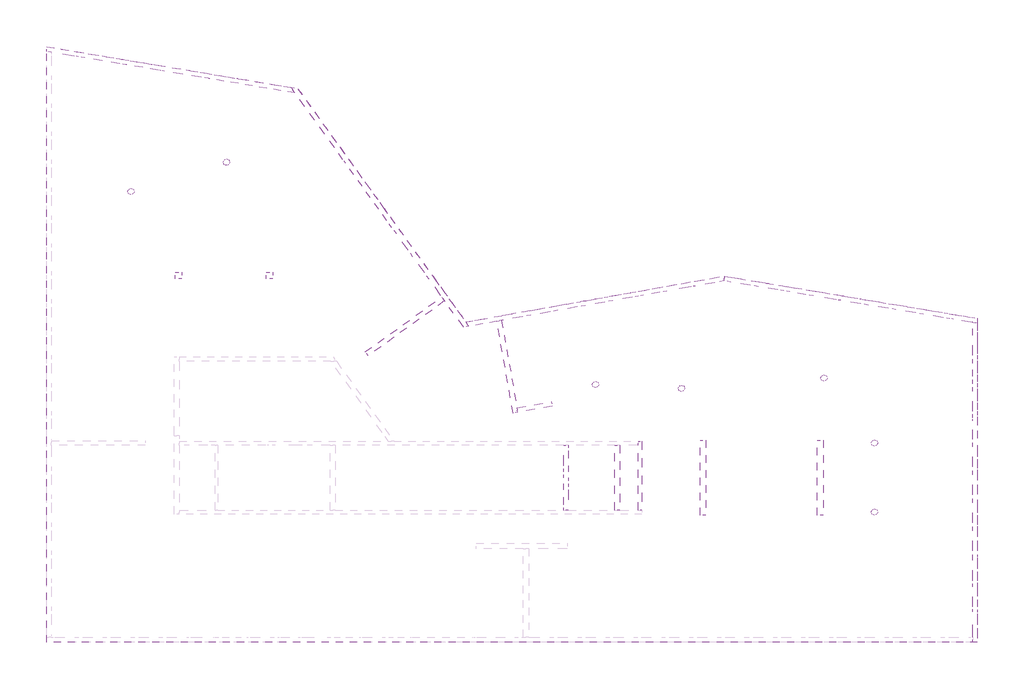
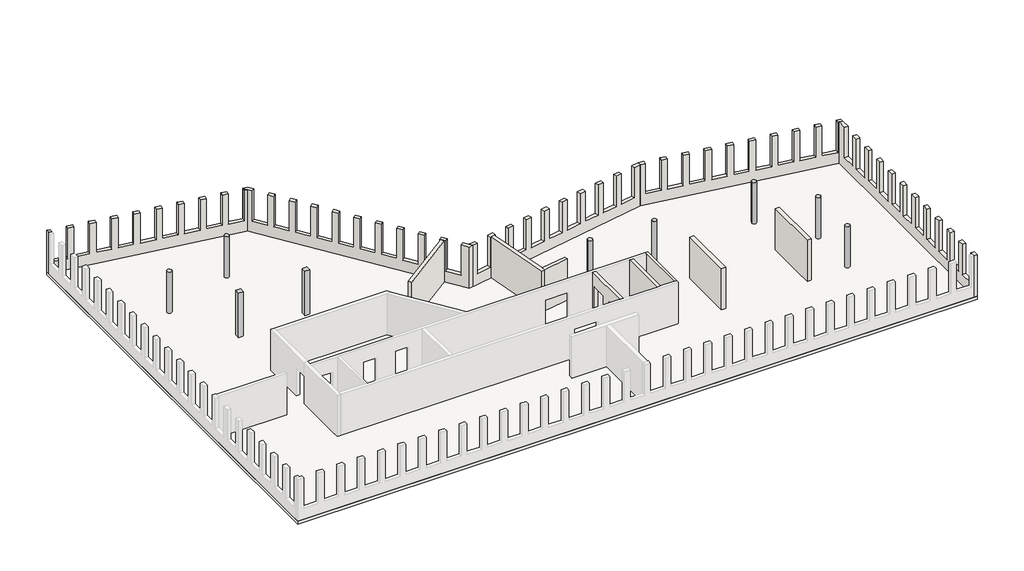
# One storey, part 2 of 2: 13 walls, 9 columns, 1 slab.
"""IFC4 building model written with IfcOpenShell, lengths in millimetres."""

from ifc_helpers import new_model, si_unit, point, frame, frame_2d, origin, place, context, project, spatial, polyline, circle_curve, trimmed, segment, composite_curve, outline, extrude, faceted_brep, element, save

model = new_model("IFC4")

# Units and contexts
model_context = context("Model", 3, world=origin())
ifc_project = project(units=[si_unit("LENGTHUNIT", "METRE", prefix="MILLI")], contexts=[model_context])

# Site, building, storey
site = spatial("IfcSite", under=ifc_project)
building = spatial("IfcBuilding", under=site)
storey = spatial("IfcBuildingStorey", under=building, Name="02_OG_OKFB_6,92", Elevation=6920.0)

# Columns
placement = place(None, origin())
element("IfcColumn", 1, ObjectType="5dki STB-Stützen rund : 5dki Stütze rund ø35cm C40/50", at=placement, inside=storey, context=model_context, shape_type="SweptSolid", body=[
    extrude(outline(composite_curve([segment(trimmed(circle_curve(frame_2d((33961.7583834, 13503.0230367)), 175.0), [point((34136.7583834, 13503.0230367))], [point((33786.7583834, 13503.0230367))], False, "CARTESIAN"), True, "CONTINUOUS"), segment(trimmed(circle_curve(frame_2d((33961.7583834, 13503.0230367)), 175.0), [point((33786.7583834, 13503.0230367))], [point((34136.7583834, 13503.0230367))], False, "CARTESIAN"), True, "CONTINUOUS")], self_intersect=False)), frame((0.0, 0.0, 10230.0), z_axis=(0.0, 0.0, 1.0), x_axis=(1.0, 0.0, 0.0)), (0.0, 0.0, 1.0), 3210.0),
])
element("IfcColumn", 2, ObjectType="5dki STB-Stützen rechteckig : 5dki Stütze recht. 35x35cm C35/45", at=placement, inside=storey, context=model_context, shape_type="SweptSolid", body=[
    extrude(outline(polyline([(7139.9999521, 19742.0124565), (7139.9999521, 19392.0124565), (6789.9999521, 19392.0124565), (6789.9999521, 19742.0124565), (7139.9999521, 19742.0124565)])), frame((0.0, 0.0, 10230.0), z_axis=(0.0, 0.0, 1.0), x_axis=(1.0, 0.0, 0.0)), (0.0, 0.0, 1.0), 3460.0),
])
element("IfcColumn", 3, ObjectType="5dki STB-Stützen rechteckig : 5dki Stütze recht. 35x35cm C35/45", at=placement, inside=storey, context=model_context, shape_type="SweptSolid", body=[
    extrude(outline(polyline([(12021.4450432, 19742.0124565), (12021.4450432, 19392.0124565), (11671.4450432, 19392.0124565), (11671.4450432, 19742.0124565), (12021.4450432, 19742.0124565)])), frame((0.0, 0.0, 10230.0), z_axis=(0.0, 0.0, 1.0), x_axis=(1.0, 0.0, 0.0)), (0.0, 0.0, 1.0), 3460.0),
])
element("IfcColumn", 4, ObjectType="5dki STB-Stützen rund : 5dki Stütze rund ø35cm C40/50", at=placement, inside=storey, context=model_context, shape_type="SweptSolid", body=[
    extrude(outline(composite_curve([segment(trimmed(circle_curve(frame_2d((41616.0718251, 14052.9332427)), 175.0), [point((41791.0718251, 14052.9332427))], [point((41441.0718251, 14052.9332427))], False, "CARTESIAN"), True, "CONTINUOUS"), segment(trimmed(circle_curve(frame_2d((41616.0718251, 14052.9332427)), 175.0), [point((41441.0718251, 14052.9332427))], [point((41791.0718251, 14052.9332427))], False, "CARTESIAN"), True, "CONTINUOUS")], self_intersect=False)), frame((0.0, 0.0, 10230.0), z_axis=(0.0, 0.0, 1.0), x_axis=(1.0, 0.0, 0.0)), (0.0, 0.0, 1.0), 3210.0),
])
element("IfcColumn", 5, ObjectType="5dki STB-Stützen rund : 5dki Stütze rund ø35cm C40/50", at=placement, inside=storey, context=model_context, shape_type="SweptSolid", body=[
    extrude(outline(composite_curve([segment(trimmed(circle_curve(frame_2d((44328.9990923, 10566.8309986)), 175.0), [point((44503.9990923, 10566.8309986))], [point((44153.9990923, 10566.8309986))], False, "CARTESIAN"), True, "CONTINUOUS"), segment(trimmed(circle_curve(frame_2d((44328.9990923, 10566.8309986)), 175.0), [point((44153.9990923, 10566.8309986))], [point((44503.9990923, 10566.8309986))], False, "CARTESIAN"), True, "CONTINUOUS")], self_intersect=False)), frame((0.0, 0.0, 10230.0), z_axis=(0.0, 0.0, 1.0), x_axis=(1.0, 0.0, 0.0)), (0.0, 0.0, 1.0), 3210.0),
])
element("IfcColumn", 6, ObjectType="5dki STB-Stützen rund : 5dki Stütze rund ø35cm C40/50", at=placement, inside=storey, context=model_context, shape_type="SweptSolid", body=[
    extrude(outline(composite_curve([segment(trimmed(circle_curve(frame_2d((44328.9990923, 6852.1619165)), 175.0), [point((44503.9990923, 6852.1619165))], [point((44153.9990923, 6852.1619165))], False, "CARTESIAN"), True, "CONTINUOUS"), segment(trimmed(circle_curve(frame_2d((44328.9990923, 6852.1619165)), 175.0), [point((44153.9990923, 6852.1619165))], [point((44503.9990923, 6852.1619165))], False, "CARTESIAN"), True, "CONTINUOUS")], self_intersect=False)), frame((0.0, 0.0, 10230.0), z_axis=(0.0, 0.0, 1.0), x_axis=(1.0, 0.0, 0.0)), (0.0, 0.0, 1.0), 3210.0),
])
element("IfcColumn", 7, ObjectType="5dki STB-Stützen rund : 5dki Stütze rund ø35cm C40/50", at=placement, inside=storey, context=model_context, shape_type="SweptSolid", body=[
    extrude(outline(composite_curve([segment(trimmed(circle_curve(frame_2d((9535.2710874, 25643.9282611)), 175.0), [point((9710.2710874, 25643.9282611))], [point((9360.2710874, 25643.9282611))], False, "CARTESIAN"), True, "CONTINUOUS"), segment(trimmed(circle_curve(frame_2d((9535.2710874, 25643.9282611)), 175.0), [point((9360.2710874, 25643.9282611))], [point((9710.2710874, 25643.9282611))], False, "CARTESIAN"), True, "CONTINUOUS")], self_intersect=False)), frame((0.0, 0.0, 10230.0), z_axis=(0.0, 0.0, 1.0), x_axis=(1.0, 0.0, 0.0)), (0.0, 0.0, 1.0), 3210.0),
])
element("IfcColumn", 8, ObjectType="5dki STB-Stützen rund : 5dki Stütze rund ø35cm C40/50", at=placement, inside=storey, context=model_context, shape_type="SweptSolid", body=[
    extrude(outline(composite_curve([segment(trimmed(circle_curve(frame_2d((4404.9034618, 24066.2757931)), 175.0), [point((4579.9034618, 24066.2757931))], [point((4229.9034618, 24066.2757931))], False, "CARTESIAN"), True, "CONTINUOUS"), segment(trimmed(circle_curve(frame_2d((4404.9034618, 24066.2757931)), 175.0), [point((4229.9034618, 24066.2757931))], [point((4579.9034618, 24066.2757931))], False, "CARTESIAN"), True, "CONTINUOUS")], self_intersect=False)), frame((0.0, 0.0, 10230.0), z_axis=(0.0, 0.0, 1.0), x_axis=(1.0, 0.0, 0.0)), (0.0, 0.0, 1.0), 3210.0),
])
element("IfcColumn", 9, ObjectType="5dki STB-Stützen rund : 5dki Stütze rund ø35cm C40/50", at=placement, inside=storey, context=model_context, shape_type="SweptSolid", body=[
    extrude(outline(composite_curve([segment(trimmed(circle_curve(frame_2d((29357.7423112, 13702.251654)), 175.0), [point((29532.7423112, 13702.251654))], [point((29182.7423112, 13702.251654))], False, "CARTESIAN"), True, "CONTINUOUS"), segment(trimmed(circle_curve(frame_2d((29357.7423112, 13702.251654)), 175.0), [point((29182.7423112, 13702.251654))], [point((29532.7423112, 13702.251654))], False, "CARTESIAN"), True, "CONTINUOUS")], self_intersect=False)), frame((0.0, 0.0, 10230.0), z_axis=(0.0, 0.0, 1.0), x_axis=(1.0, 0.0, 0.0)), (0.0, 0.0, 1.0), 3210.0),
])

# Slab
element("IfcSlab", 10, ObjectType="5dki Decke Ortbeton 25cm C30/37", at=placement, inside=storey, context=model_context, shape_type="SweptSolid", body=[
    extrude(outline(polyline([(-129.9989953, 31855.7150729), (13359.8955383, 29603.0549033), (22383.5041721, 17069.4128529), (36259.9888873, 19532.5499737), (49863.9990833, 17260.8337794), (49863.9991105, -129.9989509), (-129.9989953, -129.9990284), (-129.9989953, 31855.7150729)]), holes=[polyline([(30391.9999891, 10442.0127433), (27891.9999829, 10442.0127433), (27891.9999829, 6960.0000497), (30391.9999891, 6960.0000497), (30391.9999891, 10442.0127433)]), polyline([(31641.9999382, 10442.0127483), (30641.9999891, 10442.0127483), (30641.9999891, 6960.0000514), (31641.9999382, 6960.0000514), (31641.9999382, 10442.0127483)]), polyline([(8916.9999886, 10442.0127052), (6989.9995723, 10442.0127052), (6989.9995723, 6960.0000232), (8916.9999886, 6960.0000232), (8916.9999886, 10442.0127052)]), polyline([(24127.0004657, 8820.0328918), (16927.0004692, 8820.0328918), (16927.0004692, 7020.033352), (24127.0004657, 7020.033352), (24127.0004657, 8820.0328918)])]), frame((0.0, 0.0, 9980.0), z_axis=(0.0, 0.0, 1.0), x_axis=(1.0, 0.0, 0.0)), (0.0, 0.0, 1.0), 250.0),
])

# Walls
element("IfcWall", 11, ObjectType="5dki Lochfassade 26cm C30/37", at=placement, inside=storey, context=model_context, shape_type="Brep", body=[
    faceted_brep([(12995.7423601, 29663.864375, 10230.0), (13211.4553837, 29364.2425792, 10230.0), (22268.004401, 16784.8468851, 10230.0), (22268.004401, 16784.8468851, 13440.0), (21924.4906268, 17261.9817942, 13440.0), (21924.4906268, 17261.9817942, 11090.0), (21293.4697845, 18138.4592307, 11090.0), (21293.4697845, 18138.4592307, 13440.0), (21048.0727903, 18479.3115671, 13440.0), (21048.0727903, 18479.3115671, 11090.0), (20417.0519481, 19355.7890035, 11090.0), (20417.0519481, 19355.7890035, 13440.0), (20171.6549538, 19696.64134, 13440.0), (20171.6549538, 19696.64134, 11090.0), (19540.6341116, 20573.1187764, 11090.0), (19540.6341116, 20573.1187764, 13440.0), (19295.2371174, 20913.9711128, 13440.0), (19295.2371174, 20913.9711128, 11090.0), (18664.2162751, 21790.4485493, 11090.0), (18664.2162751, 21790.4485493, 13440.0), (18418.8192809, 22131.3008857, 13440.0), (18418.8192809, 22131.3008857, 11090.0), (17787.7984387, 23007.7783222, 11090.0), (17787.7984387, 23007.7783222, 13440.0), (17542.4014445, 23348.6306586, 13440.0), (17542.4014445, 23348.6306586, 11090.0), (16911.3806022, 24225.1080951, 11090.0), (16911.3806022, 24225.1080951, 13440.0), (16665.983608, 24565.9604315, 13440.0), (16665.983608, 24565.9604315, 11090.0), (16034.9627658, 25442.4378679, 11090.0), (16034.9627658, 25442.4378679, 13440.0), (15789.5657715, 25783.2902043, 13440.0), (15789.5657715, 25783.2902043, 11090.0), (15158.5449293, 26659.7676408, 11090.0), (15158.5449293, 26659.7676408, 13440.0), (14913.1479351, 27000.6199772, 13440.0), (14913.1479351, 27000.6199772, 11090.0), (14282.1270928, 27877.0974137, 11090.0), (14282.1270928, 27877.0974137, 13440.0), (14036.7300986, 28217.9497501, 13440.0), (14036.7300986, 28217.9497501, 11090.0), (13405.7092564, 29094.4271866, 11090.0), (13405.7092564, 29094.4271866, 13440.0), (13211.4553837, 29364.2425792, 13440.0), (13028.1664453, 29618.8278609, 13440.0), (13028.1664453, 29618.8278609, 11090.0), (12995.7423601, 29663.864375, 11090.0), (22552.0750732, 16835.2706799, 10230.0), (22383.5041721, 17069.4128529, 10230.0), (13359.8955383, 29603.0549033, 10230.0), (13359.8955383, 29603.0549033, 13440.0), (13616.7130837, 29246.3396115, 13440.0), (13616.7130837, 29246.3396115, 11090.0), (14247.7339259, 28369.8621751, 11090.0), (14247.7339259, 28369.8621751, 13440.0), (14493.1309201, 28029.0098387, 13440.0), (14493.1309201, 28029.0098387, 11090.0), (15124.1517624, 27152.5324022, 11090.0), (15124.1517624, 27152.5324022, 13440.0), (15369.5487566, 26811.6800658, 13440.0), (15369.5487566, 26811.6800658, 11090.0), (16000.5695988, 25935.2026293, 11090.0), (16000.5695988, 25935.2026293, 13440.0), (16245.966593, 25594.3502929, 13440.0), (16245.966593, 25594.3502929, 11090.0), (16876.9874353, 24717.8728564, 11090.0), (16876.9874353, 24717.8728564, 13440.0), (17122.3844295, 24377.02052, 13440.0), (17122.3844295, 24377.02052, 11090.0), (17753.4052718, 23500.5430836, 11090.0), (17753.4052718, 23500.5430836, 13440.0), (17998.802266, 23159.6907472, 13440.0), (17998.802266, 23159.6907472, 11090.0), (18629.8231082, 22283.2133107, 11090.0), (18629.8231082, 22283.2133107, 13440.0), (18875.2201024, 21942.3609743, 13440.0), (18875.2201024, 21942.3609743, 11090.0), (19506.2409447, 21065.8835378, 11090.0), (19506.2409447, 21065.8835378, 13440.0), (19751.6379389, 20725.0312014, 13440.0), (19751.6379389, 20725.0312014, 11090.0), (20382.6587811, 19848.5537649, 11090.0), (20382.6587811, 19848.5537649, 13440.0), (20628.0557754, 19507.7014285, 13440.0), (20628.0557754, 19507.7014285, 11090.0), (21259.0766176, 18631.2239921, 11090.0), (21259.0766176, 18631.2239921, 13440.0), (21504.4736118, 18290.3716557, 13440.0), (21504.4736118, 18290.3716557, 11090.0), (22135.4944541, 17413.8942192, 11090.0), (22135.4944541, 17413.8942192, 13440.0), (22383.5041721, 17069.4128529, 13440.0), (22552.0750732, 16835.2706799, 13440.0), (13034.6033862, 29657.3750221, 13440.0), (13034.6033862, 29657.3750221, 11090.0)], [[[0, 1, 2, 3, 4, 5, 6, 7, 8, 9, 10, 11, 12, 13, 14, 15, 16, 17, 18, 19, 20, 21, 22, 23, 24, 25, 26, 27, 28, 29, 30, 31, 32, 33, 34, 35, 36, 37, 38, 39, 40, 41, 42, 43, 44, 45, 46, 47]], [[48, 49, 50, 51, 52, 53, 54, 55, 56, 57, 58, 59, 60, 61, 62, 63, 64, 65, 66, 67, 68, 69, 70, 71, 72, 73, 74, 75, 76, 77, 78, 79, 80, 81, 82, 83, 84, 85, 86, 87, 88, 89, 90, 91, 92, 93]], [[2, 1, 0, 50, 49, 48]], [[3, 93, 92, 91, 4]], [[52, 51, 94, 45, 44, 43]], [[55, 40, 39, 56]], [[59, 36, 35, 60]], [[63, 32, 31, 64]], [[67, 28, 27, 68]], [[71, 24, 23, 72]], [[75, 20, 19, 76]], [[79, 16, 15, 80]], [[83, 12, 11, 84]], [[87, 8, 7, 88]], [[3, 2, 48, 93]], [[42, 53, 52, 43]], [[54, 41, 40, 55]], [[53, 42, 41, 54]], [[39, 38, 57, 56]], [[37, 36, 59, 58]], [[38, 37, 58, 57]], [[35, 34, 61, 60]], [[33, 32, 63, 62]], [[34, 33, 62, 61]], [[31, 30, 65, 64]], [[29, 28, 67, 66]], [[30, 29, 66, 65]], [[27, 26, 69, 68]], [[25, 24, 71, 70]], [[26, 25, 70, 69]], [[23, 22, 73, 72]], [[21, 20, 75, 74]], [[22, 21, 74, 73]], [[19, 18, 77, 76]], [[17, 16, 79, 78]], [[18, 17, 78, 77]], [[15, 14, 81, 80]], [[13, 12, 83, 82]], [[14, 13, 82, 81]], [[11, 10, 85, 84]], [[9, 8, 87, 86]], [[10, 9, 86, 85]], [[7, 6, 89, 88]], [[5, 4, 91, 90]], [[6, 5, 90, 89]], [[51, 50, 0, 47, 95, 94]], [[95, 46, 45, 94]], [[46, 95, 47]]]),
])
element("IfcWall", 12, ObjectType="5dki Lochfassade 26cm C30/37", at=placement, inside=storey, context=model_context, shape_type="Brep", body=[
    faceted_brep([(27318.6765704, 17681.3634281, 13440.0), (26924.8330267, 17611.4544654, 13440.0), (26924.8330267, 17611.4544654, 11090.0), (25861.4554587, 17422.7002661, 11090.0), (25861.4554587, 17422.7002661, 13440.0), (25447.9197377, 17349.2958553, 13440.0), (25447.9197377, 17349.2958553, 11090.0), (24384.5421697, 17160.541656, 11090.0), (24384.5421697, 17160.541656, 13440.0), (24300.8505369, 17145.6860228, 13440.0), (24054.698322, 17101.9929211, 13440.0), (23971.0064488, 17087.1372452, 13440.0), (23971.0064488, 17087.1372452, 11090.0), (22907.6288807, 16898.3830459, 11090.0), (22907.6288807, 16898.3830459, 13440.0), (22552.0750732, 16835.2706799, 13440.0), (22552.0750732, 16835.2706799, 10230.0), (24054.698322, 17101.9929211, 10230.0), (24300.8505369, 17145.6860228, 10230.0), (36261.33607, 19268.7248546, 10230.0), (36261.33607, 19268.7248546, 13440.0), (35766.6205834, 19180.910678, 13440.0), (35766.6205834, 19180.910678, 11090.0), (34703.2430153, 18992.1564787, 11090.0), (34703.2430153, 18992.1564787, 13440.0), (34289.7072944, 18918.7520679, 13440.0), (34289.7072944, 18918.7520679, 11090.0), (33226.3297263, 18729.9978686, 11090.0), (33226.3297263, 18729.9978686, 13440.0), (32812.7940054, 18656.5934577, 13440.0), (32812.7940054, 18656.5934577, 11090.0), (31749.4164374, 18467.8392585, 11090.0), (31749.4164374, 18467.8392585, 13440.0), (31335.8807164, 18394.4348476, 13440.0), (31335.8807164, 18394.4348476, 11090.0), (30272.5031484, 18205.6806483, 11090.0), (30272.5031484, 18205.6806483, 13440.0), (29858.9674275, 18132.2762375, 13440.0), (29858.9674275, 18132.2762375, 11090.0), (28795.5898594, 17943.5220382, 11090.0), (28795.5898594, 17943.5220382, 13440.0), (28382.0541385, 17870.1176274, 13440.0), (28382.0541385, 17870.1176274, 11090.0), (27318.6765704, 17681.3634281, 11090.0), (26879.392201, 17867.4527688, 11090.0), (26879.392201, 17867.4527688, 13440.0), (27273.2357447, 17937.3617315, 13440.0), (27273.2357447, 17937.3617315, 11090.0), (28336.6133127, 18126.1159308, 11090.0), (28336.6133127, 18126.1159308, 13440.0), (28750.1490337, 18199.5203416, 13440.0), (28750.1490337, 18199.5203416, 11090.0), (29813.5266017, 18388.2745409, 11090.0), (29813.5266017, 18388.2745409, 13440.0), (30227.0623226, 18461.6789518, 13440.0), (30227.0623226, 18461.6789518, 11090.0), (31290.4398907, 18650.433151, 11090.0), (31290.4398907, 18650.433151, 13440.0), (31703.9756116, 18723.8375619, 13440.0), (31703.9756116, 18723.8375619, 11090.0), (32767.3531797, 18912.5917612, 11090.0), (32767.3531797, 18912.5917612, 13440.0), (33180.8889006, 18985.996172, 13440.0), (33180.8889006, 18985.996172, 11090.0), (34244.2664686, 19174.7503713, 11090.0), (34244.2664686, 19174.7503713, 13440.0), (34657.8021895, 19248.1547821, 13440.0), (34657.8021895, 19248.1547821, 11090.0), (35721.1797576, 19436.9089814, 11090.0), (35721.1797576, 19436.9089814, 13440.0), (36259.9888873, 19532.5499737, 13440.0), (36259.9888873, 19532.5499737, 10230.0), (22383.5041721, 17069.4128529, 10230.0), (22383.5041721, 17069.4128529, 13440.0), (22862.188055, 17154.3813493, 13440.0), (22862.188055, 17154.3813493, 11090.0), (23925.565623, 17343.1355486, 11090.0), (23925.565623, 17343.1355486, 13440.0), (24339.1013439, 17416.5399594, 13440.0), (24339.1013439, 17416.5399594, 11090.0), (25402.478912, 17605.2941587, 11090.0), (25402.478912, 17605.2941587, 13440.0), (25816.0146329, 17678.6985695, 13440.0), (25816.0146329, 17678.6985695, 11090.0)], [[[0, 1, 2, 3, 4, 5, 6, 7, 8, 9, 10, 11, 12, 13, 14, 15, 16, 17, 18, 19, 20, 21, 22, 23, 24, 25, 26, 27, 28, 29, 30, 31, 32, 33, 34, 35, 36, 37, 38, 39, 40, 41, 42, 43]], [[44, 45, 46, 47, 48, 49, 50, 51, 52, 53, 54, 55, 56, 57, 58, 59, 60, 61, 62, 63, 64, 65, 66, 67, 68, 69, 70, 71, 72, 73, 74, 75, 76, 77, 78, 79, 80, 81, 82, 83]], [[19, 18, 17, 16, 72, 71]], [[74, 73, 15, 14]], [[50, 49, 41, 40]], [[37, 36, 54, 53]], [[58, 57, 33, 32]], [[29, 28, 62, 61]], [[21, 20, 70, 69]], [[25, 24, 66, 65]], [[78, 77, 11, 10, 9, 8]], [[82, 81, 5, 4]], [[46, 45, 1, 0]], [[16, 15, 73, 72]], [[20, 19, 71, 70]], [[14, 13, 75, 74]], [[12, 11, 77, 76]], [[13, 12, 76, 75]], [[49, 48, 42, 41]], [[47, 46, 0, 43]], [[48, 47, 43, 42]], [[40, 39, 51, 50]], [[38, 37, 53, 52]], [[39, 38, 52, 51]], [[57, 56, 34, 33]], [[55, 54, 36, 35]], [[56, 55, 35, 34]], [[32, 31, 59, 58]], [[30, 29, 61, 60]], [[31, 30, 60, 59]], [[65, 64, 26, 25]], [[63, 62, 28, 27]], [[64, 63, 27, 26]], [[69, 68, 22, 21]], [[67, 66, 24, 23]], [[68, 67, 23, 22]], [[8, 7, 79, 78]], [[6, 5, 81, 80]], [[7, 6, 80, 79]], [[4, 3, 83, 82]], [[2, 1, 45, 44]], [[3, 2, 44, 83]]]),
])
element("IfcWall", 13, ObjectType="5dki Lochfassade 26cm C30/37_f", at=placement, inside=storey, context=model_context, shape_type="Brep", body=[
    faceted_brep([(49863.9990837, 16997.2336245, 13440.0), (49603.9990837, 17040.6506907, 13440.0), (49507.8677901, 17056.7035319, 13440.0), (49507.8677901, 17056.7035319, 11090.0), (48442.6180365, 17234.5882205, 11090.0), (48442.6180365, 17234.5882205, 13440.0), (48028.3542434, 17303.7655993, 13440.0), (48028.3542434, 17303.7655993, 11090.0), (46963.1044898, 17481.6502878, 11090.0), (46963.1044898, 17481.6502878, 13440.0), (46548.8406967, 17550.8276667, 13440.0), (46548.8406967, 17550.8276667, 11090.0), (45483.5909431, 17728.7123552, 11090.0), (45483.5909431, 17728.7123552, 13440.0), (45069.32715, 17797.8897341, 13440.0), (45069.32715, 17797.8897341, 11090.0), (44004.0773964, 17975.7744226, 11090.0), (44004.0773964, 17975.7744226, 13440.0), (43589.8136033, 18044.9518015, 13440.0), (43589.8136033, 18044.9518015, 11090.0), (42524.5638497, 18222.83649, 11090.0), (42524.5638497, 18222.83649, 13440.0), (42110.3000566, 18292.0138689, 13440.0), (42110.3000566, 18292.0138689, 11090.0), (41045.050303, 18469.8985574, 11090.0), (41045.050303, 18469.8985574, 13440.0), (40630.7865099, 18539.0759362, 13440.0), (40630.7865099, 18539.0759362, 11090.0), (39565.5367563, 18716.9606248, 11090.0), (39565.5367563, 18716.9606248, 13440.0), (39151.2729632, 18786.1380036, 13440.0), (39151.2729632, 18786.1380036, 11090.0), (38086.0232096, 18964.0226921, 11090.0), (38086.0232096, 18964.0226921, 13440.0), (37671.7594165, 19033.200071, 13440.0), (37671.7594165, 19033.200071, 11090.0), (36606.5096629, 19211.0847595, 11090.0), (36606.5096629, 19211.0847595, 13440.0), (36261.33607, 19268.7248546, 13440.0), (36261.33607, 19268.7248546, 10230.0), (49603.9990837, 17040.6506907, 10230.0), (49863.9990837, 16997.2336245, 10230.0), (49550.6918818, 17313.1525467, 11090.0), (49550.6918818, 17313.1525467, 13440.0), (49863.9990833, 17260.8337794, 13440.0), (49863.9990833, 17260.8337794, 10230.0), (36259.9888873, 19532.5499737, 10230.0), (36259.9888873, 19532.5499737, 13440.0), (36649.3337546, 19467.5337743, 13440.0), (36649.3337546, 19467.5337743, 11090.0), (37714.5835082, 19289.6490858, 11090.0), (37714.5835082, 19289.6490858, 13440.0), (38128.8473013, 19220.4717069, 13440.0), (38128.8473013, 19220.4717069, 11090.0), (39194.0970549, 19042.5870184, 11090.0), (39194.0970549, 19042.5870184, 13440.0), (39608.360848, 18973.4096395, 13440.0), (39608.360848, 18973.4096395, 11090.0), (40673.6106016, 18795.524951, 11090.0), (40673.6106016, 18795.524951, 13440.0), (41087.8743947, 18726.3475721, 13440.0), (41087.8743947, 18726.3475721, 11090.0), (42153.1241483, 18548.4628836, 11090.0), (42153.1241483, 18548.4628836, 13440.0), (42567.3879414, 18479.2855048, 13440.0), (42567.3879414, 18479.2855048, 11090.0), (43632.637695, 18301.4008162, 11090.0), (43632.637695, 18301.4008162, 13440.0), (44046.9014881, 18232.2234374, 13440.0), (44046.9014881, 18232.2234374, 11090.0), (45112.1512417, 18054.3387489, 11090.0), (45112.1512417, 18054.3387489, 13440.0), (45526.4150348, 17985.16137, 13440.0), (45526.4150348, 17985.16137, 11090.0), (46591.6647884, 17807.2766815, 11090.0), (46591.6647884, 17807.2766815, 13440.0), (47005.9285815, 17738.0993026, 13440.0), (47005.9285815, 17738.0993026, 11090.0), (48071.1783351, 17560.2146141, 11090.0), (48071.1783351, 17560.2146141, 13440.0), (48485.4421282, 17491.0372352, 13440.0), (48485.4421282, 17491.0372352, 11090.0)], [[[0, 1, 2, 3, 4, 5, 6, 7, 8, 9, 10, 11, 12, 13, 14, 15, 16, 17, 18, 19, 20, 21, 22, 23, 24, 25, 26, 27, 28, 29, 30, 31, 32, 33, 34, 35, 36, 37, 38, 39, 40, 41]], [[42, 43, 44, 45, 46, 47, 48, 49, 50, 51, 52, 53, 54, 55, 56, 57, 58, 59, 60, 61, 62, 63, 64, 65, 66, 67, 68, 69, 70, 71, 72, 73, 74, 75, 76, 77, 78, 79, 80, 81]], [[41, 40, 39, 46, 45]], [[48, 47, 38, 37]], [[52, 51, 34, 33]], [[56, 55, 30, 29]], [[60, 59, 26, 25]], [[64, 63, 22, 21]], [[68, 67, 18, 17]], [[72, 71, 14, 13]], [[76, 75, 10, 9]], [[80, 79, 6, 5]], [[44, 43, 2, 1, 0]], [[39, 38, 47, 46]], [[0, 41, 45, 44]], [[37, 36, 49, 48]], [[35, 34, 51, 50]], [[36, 35, 50, 49]], [[33, 32, 53, 52]], [[31, 30, 55, 54]], [[32, 31, 54, 53]], [[29, 28, 57, 56]], [[27, 26, 59, 58]], [[28, 27, 58, 57]], [[25, 24, 61, 60]], [[23, 22, 63, 62]], [[24, 23, 62, 61]], [[21, 20, 65, 64]], [[19, 18, 67, 66]], [[20, 19, 66, 65]], [[17, 16, 69, 68]], [[15, 14, 71, 70]], [[16, 15, 70, 69]], [[13, 12, 73, 72]], [[11, 10, 75, 74]], [[12, 11, 74, 73]], [[9, 8, 77, 76]], [[7, 6, 79, 78]], [[8, 7, 78, 77]], [[5, 4, 81, 80]], [[3, 2, 43, 42]], [[4, 3, 42, 81]]]),
])
element("IfcWall", 14, ObjectType="5dki Lochfassade 26cm C30/37", at=placement, inside=storey, context=model_context, shape_type="Brep", body=[
    faceted_brep([(49603.9991105, -129.9989514, 13440.0), (49603.9991101, 130.0010486, 13440.0), (49603.9991099, 277.0124979, 13440.0), (49603.9991099, 277.0124979, 11090.0), (49603.9991082, 1357.0124979, 11090.0), (49603.9991082, 1357.0124979, 13440.0), (49603.9991075, 1777.0124979, 13440.0), (49603.9991075, 1777.0124979, 11090.0), (49603.9991058, 2857.0124979, 11090.0), (49603.9991058, 2857.0124979, 13440.0), (49603.9991052, 3277.0124979, 13440.0), (49603.9991052, 3277.0124979, 11090.0), (49603.9991035, 4357.0124979, 11090.0), (49603.9991035, 4357.0124979, 13440.0), (49603.9991028, 4777.0124979, 13440.0), (49603.9991028, 4777.0124979, 11090.0), (49603.9991011, 5857.0124979, 11090.0), (49603.9991011, 5857.0124979, 13440.0), (49603.9991005, 6277.0124979, 13440.0), (49603.9991005, 6277.0124979, 11090.0), (49603.9990988, 7357.0124979, 11090.0), (49603.9990988, 7357.0124979, 13440.0), (49603.9990981, 7777.0124979, 13440.0), (49603.9990981, 7777.0124979, 11090.0), (49603.9990964, 8857.0124979, 11090.0), (49603.9990964, 8857.0124979, 13440.0), (49603.9990958, 9277.0124979, 13440.0), (49603.9990958, 9277.0124979, 11090.0), (49603.9990941, 10357.0124979, 11090.0), (49603.9990941, 10357.0124979, 13440.0), (49603.9990934, 10777.0124979, 13440.0), (49603.9990934, 10777.0124979, 11090.0), (49603.9990918, 11857.0124979, 11090.0), (49603.9990918, 11857.0124979, 13440.0), (49603.9990911, 12277.0124979, 13440.0), (49603.9990911, 12277.0124979, 11090.0), (49603.9990894, 13357.0124979, 11090.0), (49603.9990894, 13357.0124979, 13440.0), (49603.9990888, 13777.0124979, 13440.0), (49603.9990888, 13777.0124979, 11090.0), (49603.9990871, 14857.0124979, 11090.0), (49603.9990871, 14857.0124979, 13440.0), (49603.9990864, 15277.0124979, 13440.0), (49603.9990864, 15277.0124979, 11090.0), (49603.9990847, 16357.0124979, 11090.0), (49603.9990847, 16357.0124979, 13440.0), (49603.9990837, 17040.6506907, 13440.0), (49603.9990837, 17040.6506907, 10230.0), (49603.9991101, 130.0010486, 10230.0), (49603.9991105, -129.9989514, 10230.0), (49863.9991099, 277.0124983, 11090.0), (49863.9991099, 277.0124983, 13440.0), (49863.9991105, -129.9989509, 13440.0), (49863.9991105, -129.9989509, 10230.0), (49863.9990837, 16997.2336245, 10230.0), (49863.9990837, 16997.2336245, 13440.0), (49863.9990847, 16357.0124983, 13440.0), (49863.9990847, 16357.0124983, 11090.0), (49863.9990864, 15277.0124983, 11090.0), (49863.9990864, 15277.0124983, 13440.0), (49863.9990871, 14857.0124983, 13440.0), (49863.9990871, 14857.0124983, 11090.0), (49863.9990888, 13777.0124983, 11090.0), (49863.9990888, 13777.0124983, 13440.0), (49863.9990894, 13357.0124983, 13440.0), (49863.9990894, 13357.0124983, 11090.0), (49863.9990911, 12277.0124983, 11090.0), (49863.9990911, 12277.0124983, 13440.0), (49863.9990918, 11857.0124983, 13440.0), (49863.9990918, 11857.0124983, 11090.0), (49863.9990934, 10777.0124983, 11090.0), (49863.9990934, 10777.0124983, 13440.0), (49863.9990941, 10357.0124983, 13440.0), (49863.9990941, 10357.0124983, 11090.0), (49863.9990958, 9277.0124983, 11090.0), (49863.9990958, 9277.0124983, 13440.0), (49863.9990964, 8857.0124983, 13440.0), (49863.9990964, 8857.0124983, 11090.0), (49863.9990981, 7777.0124983, 11090.0), (49863.9990981, 7777.0124983, 13440.0), (49863.9990988, 7357.0124983, 13440.0), (49863.9990988, 7357.0124983, 11090.0), (49863.9991005, 6277.0124983, 11090.0), (49863.9991005, 6277.0124983, 13440.0), (49863.9991011, 5857.0124983, 13440.0), (49863.9991011, 5857.0124983, 11090.0), (49863.9991028, 4777.0124983, 11090.0), (49863.9991028, 4777.0124983, 13440.0), (49863.9991035, 4357.0124983, 13440.0), (49863.9991035, 4357.0124983, 11090.0), (49863.9991052, 3277.0124983, 11090.0), (49863.9991052, 3277.0124983, 13440.0), (49863.9991058, 2857.0124983, 13440.0), (49863.9991058, 2857.0124983, 11090.0), (49863.9991075, 1777.0124983, 11090.0), (49863.9991075, 1777.0124983, 13440.0), (49863.9991082, 1357.0124983, 13440.0), (49863.9991082, 1357.0124983, 11090.0)], [[[0, 1, 2, 3, 4, 5, 6, 7, 8, 9, 10, 11, 12, 13, 14, 15, 16, 17, 18, 19, 20, 21, 22, 23, 24, 25, 26, 27, 28, 29, 30, 31, 32, 33, 34, 35, 36, 37, 38, 39, 40, 41, 42, 43, 44, 45, 46, 47, 48, 49]], [[50, 51, 52, 53, 54, 55, 56, 57, 58, 59, 60, 61, 62, 63, 64, 65, 66, 67, 68, 69, 70, 71, 72, 73, 74, 75, 76, 77, 78, 79, 80, 81, 82, 83, 84, 85, 86, 87, 88, 89, 90, 91, 92, 93, 94, 95, 96, 97]], [[49, 48, 47, 54, 53]], [[55, 46, 45, 56]], [[42, 41, 60, 59]], [[38, 37, 64, 63]], [[34, 33, 68, 67]], [[30, 29, 72, 71]], [[26, 25, 76, 75]], [[22, 21, 80, 79]], [[18, 17, 84, 83]], [[14, 13, 88, 87]], [[10, 9, 92, 91]], [[96, 95, 6, 5]], [[52, 51, 2, 1, 0]], [[47, 46, 55, 54]], [[0, 49, 53, 52]], [[58, 43, 42, 59]], [[44, 57, 56, 45]], [[43, 58, 57, 44]], [[63, 62, 39, 38]], [[61, 60, 41, 40]], [[62, 61, 40, 39]], [[67, 66, 35, 34]], [[65, 64, 37, 36]], [[66, 65, 36, 35]], [[71, 70, 31, 30]], [[69, 68, 33, 32]], [[70, 69, 32, 31]], [[75, 74, 27, 26]], [[73, 72, 29, 28]], [[74, 73, 28, 27]], [[79, 78, 23, 22]], [[77, 76, 25, 24]], [[78, 77, 24, 23]], [[83, 82, 19, 18]], [[81, 80, 21, 20]], [[82, 81, 20, 19]], [[87, 86, 15, 14]], [[85, 84, 17, 16]], [[86, 85, 16, 15]], [[91, 90, 11, 10]], [[89, 88, 13, 12]], [[90, 89, 12, 11]], [[95, 94, 7, 6]], [[93, 92, 9, 8]], [[94, 93, 8, 7]], [[5, 4, 97, 96]], [[3, 2, 51, 50]], [[4, 3, 50, 97]]]),
])
element("IfcWall", 15, ObjectType="5dki STB-Wand Kern 25cm C30/37", at=placement, inside=storey, context=model_context, shape_type="SweptSolid", body=[
    extrude(outline(polyline([(30641.9999891, 10442.0127483), (30641.9999891, 6960.0000501), (30391.9999891, 6960.0000498), (30391.9999891, 10442.0127479), (30641.9999891, 10442.0127483)])), frame((0.0, 0.0, 10230.0), z_axis=(0.0, 0.0, 1.0), x_axis=(1.0, 0.0, 0.0)), (0.0, 0.0, 1.0), 3210.0),
])
element("IfcWall", 16, ObjectType="5dki STB-Wand Kern 25cm C30/37", at=placement, inside=storey, context=model_context, shape_type="SweptSolid", body=[
    extrude(outline(polyline([(3482.0126944, -3210.0), (-2.1e-06, -3210.0), (-2.1e-06, 0.0), (279.9681323, 0.0), (279.9681323, -2260.0), (1414.9681323, -2260.0), (1414.9681323, 0.0), (2067.1995869, 0.0), (2067.1995869, -2260.0), (3202.1995869, -2260.0), (3202.1995869, 0.0), (3482.0126944, 0.0), (3482.0126944, -3210.0)])), frame((27641.9999829, 10442.0127408, 10230.0), z_axis=(1.0, 1.6300916066412081e-09, 0.0), x_axis=(1.6300916066412081e-09, -1.0, 0.0)), (0.0, 0.0, 1.0), 250.0),
])
element("IfcWall", 17, ObjectType="5dki STB-Wand Kern 20cm C35/45", at=placement, inside=storey, context=model_context, shape_type="Brep", body=[
    faceted_brep([(31641.9999912, 10662.0127502, 10230.0), (31641.9999881, 10442.0127502, 10230.0), (31641.9999382, 6960.0000514, 10230.0), (31641.9999382, 6960.0000514, 13440.0), (31641.9999881, 10442.0127502, 13440.0), (31641.9999912, 10662.0127502, 13440.0), (31841.9999912, 10662.0127505, 10230.0), (31841.9999912, 10662.0127505, 13440.0), (31841.9999382, 6960.0000516, 13440.0), (31841.9999382, 6960.0000516, 10230.0)], [[[0, 1, 2, 3, 4, 5]], [[6, 7, 8, 9]], [[2, 1, 0, 6, 9]], [[5, 4, 3, 8, 7]], [[0, 5, 7, 6]], [[3, 2, 9, 8]]]),
])
element("IfcWall", 18, ObjectType="5dki Lochfassade 26cm C30/37", at=placement, inside=storey, context=model_context, shape_type="Brep", body=[
    faceted_brep([(8967.5024476, 30072.9348316, 11090.0), (8967.5024476, 30072.9348316, 13440.0), (8553.2386546, 30142.1122105, 13440.0), (8553.2386546, 30142.1122105, 11090.0), (7487.988901, 30319.9968993, 11090.0), (7487.988901, 30319.9968993, 13440.0), (7073.7251079, 30389.1742783, 13440.0), (7073.7251079, 30389.1742783, 11090.0), (6008.4753544, 30567.058967, 11090.0), (6008.4753544, 30567.058967, 13440.0), (5594.2115613, 30636.236346, 13440.0), (5594.2115613, 30636.236346, 11090.0), (4528.9618077, 30814.1210348, 11090.0), (4528.9618077, 30814.1210348, 13440.0), (4114.6980147, 30883.2984137, 13440.0), (4114.6980147, 30883.2984137, 11090.0), (3049.4482611, 31061.1831025, 11090.0), (3049.4482611, 31061.1831025, 13440.0), (2635.184468, 31130.3604815, 13440.0), (2635.184468, 31130.3604815, 11090.0), (1569.9347144, 31308.2451702, 11090.0), (1569.9347144, 31308.2451702, 13440.0), (1155.6709214, 31377.4225492, 13440.0), (1155.6709214, 31377.4225492, 11090.0), (90.4211678, 31555.307238, 11090.0), (90.4211678, 31555.307238, 13440.0), (-129.9989953, 31592.114918, 13440.0), (-129.9989953, 31592.114918, 10230.0), (130.0010047, 31548.6978518, 10230.0), (13211.4553837, 29364.2425792, 10230.0), (13211.4553837, 29364.2425792, 13440.0), (12991.7792945, 29400.9260074, 13440.0), (12991.7792945, 29400.9260074, 11090.0), (11926.5295409, 29578.8106961, 11090.0), (11926.5295409, 29578.8106961, 13440.0), (11512.2657479, 29647.9880751, 13440.0), (11512.2657479, 29647.9880751, 11090.0), (10447.0159943, 29825.8727639, 11090.0), (10447.0159943, 29825.8727639, 13440.0), (10032.7522012, 29895.0501428, 13440.0), (10032.7522012, 29895.0501428, 11090.0), (8596.0627463, 30398.5612253, 13440.0), (9010.3265394, 30329.3838463, 13440.0), (9010.3265394, 30329.3838463, 11090.0), (10075.576293, 30151.4991576, 11090.0), (10075.576293, 30151.4991576, 13440.0), (10489.840086, 30082.3217786, 13440.0), (10489.840086, 30082.3217786, 11090.0), (11555.0898396, 29904.4370898, 11090.0), (11555.0898396, 29904.4370898, 13440.0), (11969.3536327, 29835.2597109, 13440.0), (11969.3536327, 29835.2597109, 11090.0), (12995.7423601, 29663.864375, 11090.0), (12995.7423601, 29663.864375, 10230.0), (-129.9989953, 31855.7150729, 10230.0), (-129.9989953, 31855.7150729, 13440.0), (133.2452595, 31811.7562527, 13440.0), (133.2452595, 31811.7562527, 11090.0), (1198.4950131, 31633.8715639, 11090.0), (1198.4950131, 31633.8715639, 13440.0), (1612.7588062, 31564.694185, 13440.0), (1612.7588062, 31564.694185, 11090.0), (2678.0085598, 31386.8094962, 11090.0), (2678.0085598, 31386.8094962, 13440.0), (3092.2723528, 31317.6321172, 13440.0), (3092.2723528, 31317.6321172, 11090.0), (4157.5221064, 31139.7474285, 11090.0), (4157.5221064, 31139.7474285, 13440.0), (4571.7858995, 31070.5700495, 13440.0), (4571.7858995, 31070.5700495, 11090.0), (5637.035653, 30892.6853608, 11090.0), (5637.035653, 30892.6853608, 13440.0), (6051.2994461, 30823.5079818, 13440.0), (6051.2994461, 30823.5079818, 11090.0), (7116.5491997, 30645.623293, 11090.0), (7116.5491997, 30645.623293, 13440.0), (7530.8129927, 30576.4459141, 13440.0), (7530.8129927, 30576.4459141, 11090.0), (8596.0627463, 30398.5612253, 11090.0), (13028.1664453, 29618.8278609, 13440.0), (13028.1664453, 29618.8278609, 11090.0)], [[[0, 1, 2, 3, 4, 5, 6, 7, 8, 9, 10, 11, 12, 13, 14, 15, 16, 17, 18, 19, 20, 21, 22, 23, 24, 25, 26, 27, 28, 29, 30, 31, 32, 33, 34, 35, 36, 37, 38, 39, 40]], [[41, 42, 43, 44, 45, 46, 47, 48, 49, 50, 51, 52, 53, 54, 55, 56, 57, 58, 59, 60, 61, 62, 63, 64, 65, 66, 67, 68, 69, 70, 71, 72, 73, 74, 75, 76, 77, 78]], [[29, 28, 27, 54, 53]], [[49, 35, 34, 50]], [[22, 21, 60, 59]], [[18, 17, 64, 63]], [[14, 13, 68, 67]], [[10, 9, 72, 71]], [[6, 5, 76, 75]], [[39, 38, 46, 45]], [[2, 1, 42, 41]], [[31, 30, 79]], [[55, 26, 25, 56]], [[37, 47, 46, 38]], [[48, 36, 35, 49]], [[47, 37, 36, 48]], [[58, 23, 22, 59]], [[24, 57, 56, 25]], [[23, 58, 57, 24]], [[63, 62, 19, 18]], [[61, 60, 21, 20]], [[62, 61, 20, 19]], [[67, 66, 15, 14]], [[65, 64, 17, 16]], [[66, 65, 16, 15]], [[71, 70, 11, 10]], [[69, 68, 13, 12]], [[70, 69, 12, 11]], [[75, 74, 7, 6]], [[73, 72, 9, 8]], [[74, 73, 8, 7]], [[41, 78, 3, 2]], [[77, 76, 5, 4]], [[78, 77, 4, 3]], [[45, 44, 40, 39]], [[43, 42, 1, 0]], [[44, 43, 0, 40]], [[30, 29, 53, 52, 80, 79]], [[33, 51, 50, 34]], [[80, 32, 31, 79]], [[51, 33, 32, 80, 52]], [[27, 26, 55, 54]]]),
])
element("IfcWall", 19, ObjectType="5dki STB-Wand 25cm C30/37", at=placement, inside=storey, context=model_context, shape_type="SweptSolid", body=[
    extrude(outline(polyline([(16994.6178661, 15452.6713643), (21084.845921, 18397.4352698), (21230.9155592, 18194.5469734), (17140.6875043, 15249.783068), (16994.6178661, 15452.6713643)])), frame((0.0, 0.0, 10230.0), z_axis=(0.0, 0.0, 1.0), x_axis=(1.0, 0.0, 0.0)), (0.0, 0.0, 1.0), 3210.0),
])
element("IfcWall", 20, ObjectType="5dki STB-Wand 25cm C30/37", at=placement, inside=storey, context=model_context, shape_type="Brep", body=[
    faceted_brep([(24054.698322, 17101.9929211, 10230.0), (24930.952116, 12165.4742089, 10230.0), (24930.952116, 12165.4742089, 13440.0), (24054.698322, 17101.9929211, 13440.0), (24300.8505369, 17145.6860228, 10230.0), (24300.8505369, 17145.6860228, 13440.0), (25133.4112296, 12455.3195251, 13440.0), (25177.1043309, 12209.1673103, 13440.0), (25177.1043309, 12209.1673103, 10230.0), (25133.4112296, 12455.3195251, 10230.0)], [[[0, 1, 2, 3]], [[4, 5, 6, 7, 8, 9]], [[1, 0, 4, 9, 8]], [[3, 2, 7, 6, 5]], [[0, 3, 5, 4]], [[2, 1, 8, 7]]]),
])
element("IfcWall", 21, ObjectType="5dki STB-Wand 25cm C30/37", at=placement, inside=storey, context=model_context, shape_type="SweptSolid", body=[
    extrude(outline(polyline([(27026.4023238, 12537.4258416), (25177.1043309, 12209.1673103), (25133.4112296, 12455.3195251), (26982.7092225, 12783.5780565), (27026.4023238, 12537.4258416)])), frame((0.0, 0.0, 10230.0), z_axis=(0.0, 0.0, 1.0), x_axis=(1.0, 0.0, 0.0)), (0.0, 0.0, 1.0), 3210.0),
])
element("IfcWall", 22, ObjectType="5dki STB-Wand 30cm C30/37", at=placement, inside=storey, context=model_context, shape_type="SweptSolid", body=[
    extrude(outline(polyline([(34969.9990839, 6680.0000532), (34969.9990776, 10702.0125181), (35269.9990776, 10702.0125186), (35269.9990839, 6680.0000537), (34969.9990839, 6680.0000532)])), frame((0.0, 0.0, 10230.0), z_axis=(0.0, 0.0, 1.0), x_axis=(1.0, 0.0, 0.0)), (0.0, 0.0, 1.0), 3210.0),
])
element("IfcWall", 23, ObjectType="5dki STB-Wand 30cm C30/37", at=placement, inside=storey, context=model_context, shape_type="SweptSolid", body=[
    extrude(outline(polyline([(41269.9990703, 6680.000074), (41269.9990703, 10722.0122605), (41569.9990703, 10722.0122605), (41569.9990703, 6680.000074), (41269.9990703, 6680.000074)])), frame((0.0, 0.0, 10230.0), z_axis=(0.0, 0.0, 1.0), x_axis=(1.0, 0.0, 0.0)), (0.0, 0.0, 1.0), 3210.0),
])

save(model, "model.ifc")

# Revit data of these elements
# Type "5dki STB-Stützen rund : 5dki Stütze rund ø35cm C40/50"
#   cpiFitMatchKey = "5D-KI-STB-OB-ST-RUN"
#   cpiComponentType = "Column"
#   5d Materialgüte = "C40/50"
#   Radius = 0.175 m
#   Durchmesser = 0.350 m
#   5dki Bewehrung Stab kg pro m3 = 0
#   5dki Sichtbeton SB3/SB4 [instance default] = no
#   Structural Material = 5d Beton - Stahlbeton
#   Assembly Code = ""
# Type "5dki STB-Stützen rechteckig : 5dki Stütze recht. 35x35cm C35/45"
#   cpiFitMatchKey = "5D-KI-STB-OB-ST-REC"
#   cpiComponentType = "Column"
#   5d Materialgüte = "C35/45"
#   Tiefe = 0.350 m
#   Breite = 0.350 m
#   5dki Bewehrung Stab kg pro m3 = 0
#   5dki Sichtbeton SB3/SB4 [instance default] = no
#   Structural Material = 5d Beton - Stahlbeton
#   Assembly Code = ""
# Type "5dki Decke Ortbeton 25cm C30/37"
#   cpiComponentType = "Slab"
#   cpiFitMatchKey = "5D-KI-STB-OB-DE"
#   5d Materialgüte = "C30/37"
#   Function = 0
#   5dki WU = no
#   Layers, outside or top first: 0.250 m "5d Beton - Stahlbeton" (function 1)
# Type "5dki Lochfassade 26cm C30/37"
#   Type Comments = ""
#   Description = ""
#   cpiComponentType = "Wall"
#   cpiFitMatchKey = "5D-KI-STB-OB-W-LF"
#   5d Materialgüte = "C35/45"
#   Filter Tragend / Nichttragend = yes
#   5dki WU = no
#   Layers, outside or top first: 0.260 m "5d Beton - Stahlbeton" (function 1)
# Type "5dki Lochfassade 26cm C30/37_f"
#   Type Comments = ""
#   Description = ""
#   cpiComponentType = ""
#   cpiFitMatchKey = "5D-KI-STB-OB-W-LF"
#   5d Materialgüte = "C35/45"
#   Filter Tragend / Nichttragend = yes
#   5dki WU = no
#   Layers, outside or top first: 0.260 m "5d Beton - Stahlbeton" (function 1)
# Type "5dki STB-Wand Kern 25cm C30/37"
#   Type Comments = ""
#   Description = ""
#   cpiComponentType = "Wall"
#   cpiFitMatchKey = "5D-KI-STB-OB-W-K"
#   5d Materialgüte = "C30/37"
#   Filter Tragend / Nichttragend = yes
#   5dki WU = no
#   Layers, outside or top first: 0.250 m "5d Beton - Stahlbeton" (function 1)
# Type "5dki STB-Wand Kern 20cm C35/45"
#   Type Comments = ""
#   Description = ""
#   cpiComponentType = "Wall"
#   cpiFitMatchKey = "5D-KI-STB-OB-W-K"
#   5d Materialgüte = "C35/45"
#   Filter Tragend / Nichttragend = yes
#   5dki WU = no
#   Layers, outside or top first: 0.200 m "5d Beton - Stahlbeton" (function 1)
# Type "5dki STB-Wand 25cm C30/37"
#   Type Comments = ""
#   Description = ""
#   cpiComponentType = "Wall"
#   cpiFitMatchKey = "5D-KI-STB-OB-W"
#   5d Materialgüte = "C30/37"
#   Filter Tragend / Nichttragend = yes
#   5dki WU = no
#   Layers, outside or top first: 0.250 m "5d Beton - Stahlbeton" (function 1)
# Type "5dki STB-Wand 30cm C30/37"
#   Type Comments = ""
#   Description = ""
#   cpiComponentType = "Wall"
#   cpiFitMatchKey = "5D-KI-STB-OB-W"
#   5d Materialgüte = "C30/37"
#   Filter Tragend / Nichttragend = yes
#   5dki WU = no
#   Layers, outside or top first: 0.300 m "5d Beton - Stahlbeton" (function 1)
# Elements 1, 9 (IfcColumn, "5dki STB-Stützen rund : 5dki Stütze rund ø35cm C40/50")
#   Comments = ""
#   000_080_030_Geschoß = "03_OG"
#   5dki Sichtbeton SB3/SB4 = no
#   Phase Created = Neu
#   Materials on its faces: "5d Beton - Stahlbeton"
# Element 2 (IfcColumn, "5dki STB-Stützen rechteckig : 5dki Stütze recht. 35x35cm C35/45")
#   Comments = ""
#   000_080_030_Geschoß = "03_OG"
#   5dki Sichtbeton SB3/SB4 = no
#   Phase Created = Neu
#   Materials on its faces: "5d Beton - Stahlbeton"
# Element 3 (IfcColumn, "5dki STB-Stützen rechteckig : 5dki Stütze recht. 35x35cm C35/45")
#   000_080_030_Geschoß = "03_OG"
#   5dki Sichtbeton SB3/SB4 = no
#   Phase Created = Neu
#   Materials on its faces: "5d Beton - Stahlbeton"
# Elements 4, 5, 6, 7, 8 (IfcColumn, "5dki STB-Stützen rund : 5dki Stütze rund ø35cm C40/50")
#   000_080_030_Geschoß = "03_OG"
#   5dki Sichtbeton SB3/SB4 = no
#   Phase Created = Neu
#   Materials on its faces: "5d Beton - Stahlbeton"
# Element 10 (IfcSlab, "5dki Decke Ortbeton 25cm C30/37")
#   000_080_030_Geschoß = "02_OG"
#   built-in parameter 1001955 = 2.97613 (stored number, unit not read)
#   Height Offset From Level = 0.000 m
#   built-in parameter 1001954 = 1
#   Phase Created = Neu
#   Materials on its faces: "5d Beton - Stahlbeton"
# Elements 11, 12, 14, 18 (IfcWall, "5dki Lochfassade 26cm C30/37")
#   Comments = ""
#   000_080_030_Geschoß = "03_OG"
#   Top Offset = 0.000 m
#   Base Offset = 0.000 m
#   wall height = 3.210 m
#   Phase Created = Neu
#   Base Constraint = 02_OG_OKRD_10,23
#   Top Constraint = 03_OG_UKRD_13,44
#   Materials on its faces: "5d Beton - Stahlbeton"
# Element 13 (IfcWall, "5dki Lochfassade 26cm C30/37_f")
#   Comments = ""
#   000_080_030_Geschoß = "03_OG"
#   Top Offset = 0.000 m
#   Base Offset = 0.000 m
#   wall height = 3.210 m
#   Phase Created = Neu
#   Base Constraint = 02_OG_OKRD_10,23
#   Top Constraint = 03_OG_UKRD_13,44
#   Materials on its faces: "5d Beton - Stahlbeton"
# Elements 15, 16 (IfcWall, "5dki STB-Wand Kern 25cm C30/37")
#   Comments = ""
#   000_080_030_Geschoß = "03_OG"
#   Top Offset = 0.000 m
#   Base Offset = 0.000 m
#   wall height = 3.210 m
#   Phase Created = Neu
#   Base Constraint = 02_OG_OKRD_10,23
#   Top Constraint = 03_OG_UKRD_13,44
#   Materials on its faces: "5d Beton - Stahlbeton"
# Element 17 (IfcWall, "5dki STB-Wand Kern 20cm C35/45")
#   Comments = ""
#   000_080_030_Geschoß = "03_OG"
#   Top Offset = 0.000 m
#   Base Offset = 0.000 m
#   wall height = 3.210 m
#   Phase Created = Neu
#   Base Constraint = 02_OG_OKRD_10,23
#   Top Constraint = 03_OG_UKRD_13,44
#   Materials on its faces: "5d Beton - Stahlbeton"
# Elements 19, 20 (IfcWall, "5dki STB-Wand 25cm C30/37")
#   Comments = ""
#   000_080_030_Geschoß = "03_OG"
#   Top Offset = 0.000 m
#   Base Offset = 0.000 m
#   wall height = 3.210 m
#   Phase Created = Neu
#   Base Constraint = 02_OG_OKRD_10,23
#   Top Constraint = 03_OG_UKRD_13,44
#   Materials on its faces: "5d Beton - Stahlbeton"
# Element 21 (IfcWall, "5dki STB-Wand 25cm C30/37")
#   000_080_030_Geschoß = "03_OG"
#   Top Offset = 0.000 m
#   Base Offset = 0.000 m
#   wall height = 3.210 m
#   Phase Created = Neu
#   Base Constraint = 02_OG_OKRD_10,23
#   Top Constraint = 03_OG_UKRD_13,44
#   Materials on its faces: "5d Beton - Stahlbeton"
# Element 22 (IfcWall, "5dki STB-Wand 30cm C30/37")
#   000_080_030_Geschoß = "03_OG"
#   Top Offset = 0.000 m
#   Base Offset = 0.000 m
#   wall height = 3.210 m
#   Phase Created = Neu
#   Base Constraint = 02_OG_OKRD_10,23
#   Top Constraint = 03_OG_UKRD_13,44
#   Materials on its faces: "5d Beton - Stahlbeton"
# Element 23 (IfcWall, "5dki STB-Wand 30cm C30/37")
#   Comments = ""
#   000_080_030_Geschoß = "03_OG"
#   Top Offset = 0.000 m
#   Base Offset = 0.000 m
#   wall height = 3.210 m
#   Phase Created = Neu
#   Base Constraint = 02_OG_OKRD_10,23
#   Top Constraint = 03_OG_UKRD_13,44
#   Materials on its faces: "5d Beton - Stahlbeton"
# Materials
#   "5d Beton - Stahlbeton": class "5dki", colour RGB 200 200 200, transparency 0, Cost = 0
